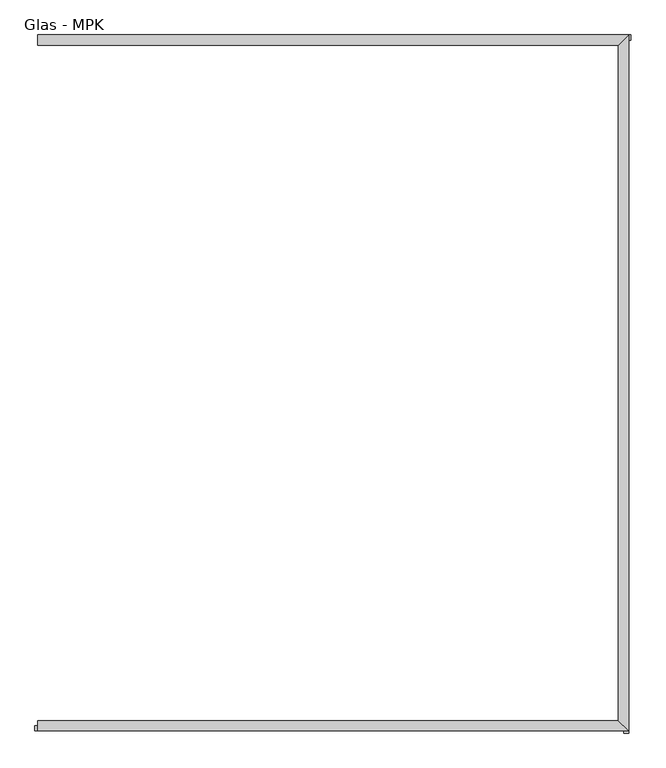
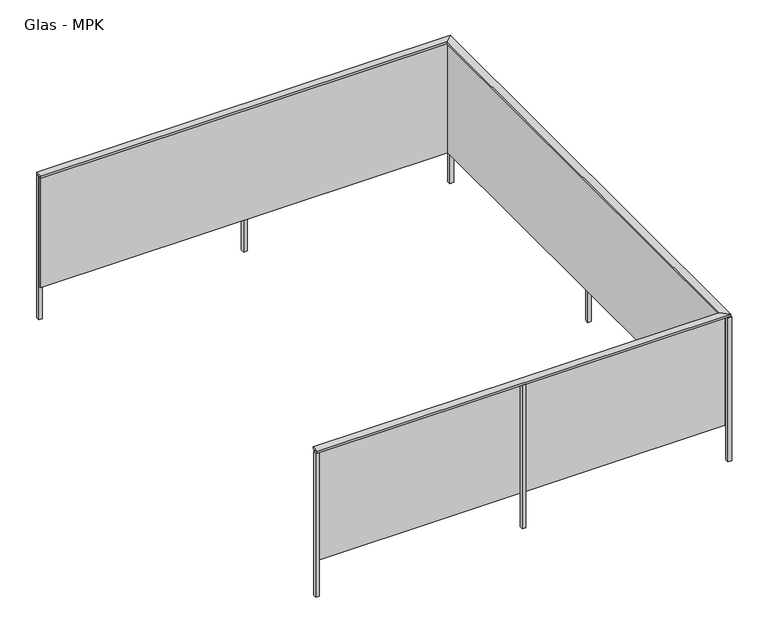
"""IFC4 building model written with IfcOpenShell, lengths in millimetres: railing geometry, Glas - MPK."""

from ifc_helpers import new_model, si_unit, frame, origin, place, context, project, spatial, polyline, outline, extrude, faceted_brep, source, transform, mapped, element, save


def glas_mpk_050cb379(model_context):
    return source(origin(), model_context, "Body", "SolidModel", [
        faceted_brep([(28820.3199184, 1288.5335867, 3843.2628643), (28820.3199184, 1238.5335867, 3843.2628643), (28820.3199184, 1238.5335867, 3856.7371357), (28820.3199184, 1288.5335867, 3856.7371357), (31660.3199184, 1288.5335867, 3843.2628643), (31610.3199184, 1238.5335867, 3843.2628643), (31610.3199184, 1238.5335867, 3856.7371357), (31660.3199184, 1288.5335867, 3856.7371357), (31660.3199184, -2052.1957594, 3843.2628643), (31610.3199184, -2002.1957594, 3843.2628643), (31610.3199184, -2002.1957594, 3856.7371357), (31660.3199184, -2052.1957594, 3856.7371357), (28820.3199184, -2052.1957594, 3843.2628643), (28820.3199184, -2052.1957594, 3856.7371357), (28820.3199184, -2002.1957594, 3856.7371357), (28820.3199184, -2002.1957594, 3843.2628643)], [[[0, 1, 2, 3]], [[1, 0, 4, 5]], [[2, 1, 5, 6]], [[3, 2, 6, 7]], [[0, 3, 7, 4]], [[5, 4, 8, 9]], [[6, 5, 9, 10]], [[7, 6, 10, 11]], [[4, 7, 11, 8]], [[12, 13, 14, 15]], [[9, 8, 12, 15]], [[10, 9, 15, 14]], [[11, 10, 14, 13]], [[8, 11, 13, 12]]]),
        faceted_brep([(28820.3199184, 1248.5335867, 3842.8769824), (28820.3199184, 1262.7257107, 3842.8769824), (28820.3199184, 1262.7257107, 3042.8769824), (28820.3199184, 1248.5335867, 3042.8769824), (31620.3199184, 1248.5335867, 3842.8769824), (31634.5120424, 1262.7257107, 3842.8769824), (31634.5120424, 1262.7257107, 3042.8769824), (31620.3199184, 1248.5335867, 3042.8769824), (31620.3199184, -2012.1957594, 3842.8769824), (31634.5120424, -2026.3878834, 3842.8769824), (31634.5120424, -2026.3878834, 3042.8769824), (31620.3199184, -2012.1957594, 3042.8769824), (28820.3199184, -2012.1957594, 3842.8769824), (28820.3199184, -2012.1957594, 3042.8769824), (28820.3199184, -2026.3878834, 3042.8769824), (28820.3199184, -2026.3878834, 3842.8769824)], [[[0, 1, 2, 3]], [[1, 0, 4, 5]], [[2, 1, 5, 6]], [[3, 2, 6, 7]], [[0, 3, 7, 4]], [[5, 4, 8, 9]], [[6, 5, 9, 10]], [[7, 6, 10, 11]], [[4, 7, 11, 8]], [[12, 13, 14, 15]], [[9, 8, 12, 15]], [[10, 9, 15, 14]], [[11, 10, 14, 13]], [[8, 11, 13, 12]]]),
        extrude(outline(polyline([(30251.5699184, -2027.1957594), (30251.5699184, -2052.1957594), (30226.5699184, -2052.1957594), (30226.5699184, -2027.1957594), (30251.5699184, -2027.1957594)])), frame((0.0, 0.0, 2800.0), z_axis=(0.0, 0.0, 1.0), x_axis=(1.0, 0.0, 0.0)), (0.0, 0.0, 1.0), 1043.2628643),
        extrude(outline(polyline([(31635.3199184, -369.3310864), (31660.3199184, -369.3310864), (31660.3199184, -394.3310864), (31635.3199184, -394.3310864), (31635.3199184, -369.3310864)])), frame((0.0, 0.0, 2800.0), z_axis=(0.0, 0.0, 1.0), x_axis=(1.0, 0.0, 0.0)), (0.0, 0.0, 1.0), 1043.2628643),
        extrude(outline(polyline([(30226.5699184, 1263.5335867), (30226.5699184, 1288.5335867), (30251.5699184, 1288.5335867), (30251.5699184, 1263.5335867), (30226.5699184, 1263.5335867)])), frame((0.0, 0.0, 2800.0), z_axis=(0.0, 0.0, 1.0), x_axis=(1.0, 0.0, 0.0)), (0.0, 0.0, 1.0), 1043.2628643),
        extrude(outline(polyline([(31635.3199184, -2037.1957594), (31660.3199184, -2037.1957594), (31660.3199184, -2062.1957594), (31635.3199184, -2062.1957594), (31635.3199184, -2037.1957594)])), frame((0.0, 0.0, 2800.0), z_axis=(0.0, 0.0, 1.0), x_axis=(1.0, 0.0, 0.0)), (0.0, 0.0, 1.0), 1043.2628643),
        extrude(outline(polyline([(31645.3199184, 1263.5335867), (31645.3199184, 1288.5335867), (31670.3199184, 1288.5335867), (31670.3199184, 1263.5335867), (31645.3199184, 1263.5335867)])), frame((0.0, 0.0, 2800.0), z_axis=(0.0, 0.0, 1.0), x_axis=(1.0, 0.0, 0.0)), (0.0, 0.0, 1.0), 1043.2628643),
        extrude(outline(polyline([(28832.8199184, -2027.1957594), (28832.8199184, -2052.1957594), (28807.8199184, -2052.1957594), (28807.8199184, -2027.1957594), (28832.8199184, -2027.1957594)])), frame((0.0, 0.0, 2800.0), z_axis=(0.0, 0.0, 1.0), x_axis=(1.0, 0.0, 0.0)), (0.0, 0.0, 1.0), 1043.2628643),
        extrude(outline(polyline([(28820.3199184, 1263.5335867), (28820.3199184, 1288.5335867), (28845.3199184, 1288.5335867), (28845.3199184, 1263.5335867), (28820.3199184, 1263.5335867)])), frame((0.0, 0.0, 2800.0), z_axis=(0.0, 0.0, 1.0), x_axis=(1.0, 0.0, 0.0)), (0.0, 0.0, 1.0), 1043.2628643),
    ])


if __name__ == "__main__":
    model = new_model("IFC4")
    model_context = context("Model", 3, world=origin())
    ifc_project = project(units=[si_unit("LENGTHUNIT", "METRE", prefix="MILLI")], contexts=[model_context])
    site = spatial("IfcSite", under=ifc_project)
    building = spatial("IfcBuilding", under=site)
    placement = place(None, origin())
    glas_mpk_shape = glas_mpk_050cb379(model_context)
    element("IfcRailing", 1, ObjectType="Glas - MPK", at=placement, inside=building, context=model_context, shape_type="MappedRepresentation", body=[
        mapped(glas_mpk_shape, transform((0.0, 0.0, 0.0), x_axis=(1.0, 0.0, 0.0), y_axis=(0.0, 1.0, 0.0), z_axis=(0.0, 0.0, 1.0))),
    ])
    save(model, "model.ifc")

# Revit data of these elements
# Element 1 (IfcRailing, "Glas - MPK")
#   Materials on its faces: "Metal - Aluminum", "Window - Glass"
# Materials
#   "Metal - Aluminum": class "Unassigned", colour RGB 247 247 247, transparency 0, Comments = "Rendering appearance not upgraded "
#   "Window - Glass": class "Glas", colour RGB 128 128 255, transparency 0.75
